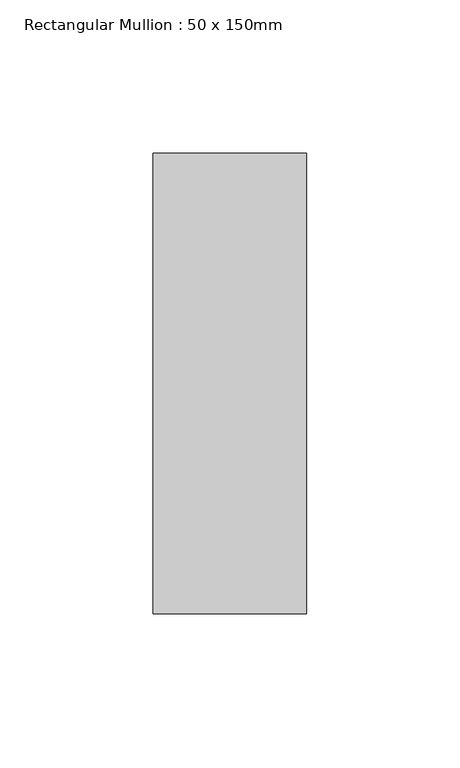
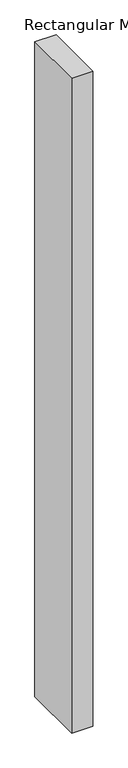
"""IFC4 building model written with IfcOpenShell, lengths in millimetres: member geometry, Rectangular Mullion : 50 x 150mm."""

from ifc_helpers import new_model, si_unit, frame, origin, place, context, project, spatial, polyline, outline, extrude, source, transform, mapped, element, save


def rectangular_mullion_50_x_150mm_9bc3b149(model_context):
    return source(origin(), model_context, "Body", "SweptSolid", [
        extrude(outline(polyline([(25.0, 75.0), (25.0, -75.0), (-25.0, -75.0), (-25.0, 75.0), (25.0, 75.0)])), frame((0.0, 0.0, -1635.0991456), z_axis=(0.0, 0.0, 1.0), x_axis=(1.0, 0.0, 0.0)), (0.0, 0.0, 1.0), 1635.0991456),
    ])


if __name__ == "__main__":
    model = new_model("IFC4")
    model_context = context("Model", 3, world=origin())
    ifc_project = project(units=[si_unit("LENGTHUNIT", "METRE", prefix="MILLI")], contexts=[model_context])
    site = spatial("IfcSite", under=ifc_project)
    building = spatial("IfcBuilding", under=site)
    placement = place(None, origin())
    rectangular_mullion_50_x_150mm_shape = rectangular_mullion_50_x_150mm_9bc3b149(model_context)
    element("IfcMember", 1, ObjectType="Rectangular Mullion : 50 x 150mm", at=placement, inside=building, context=model_context, shape_type="MappedRepresentation", body=[
        mapped(rectangular_mullion_50_x_150mm_shape, transform((0.0, 0.0, 0.0), x_axis=(1.0, 0.0, 0.0), y_axis=(0.0, 1.0, 0.0), z_axis=(0.0, 0.0, 1.0))),
    ])
    save(model, "model.ifc")

# Revit data of these elements
# Type "Rectangular Mullion : 50 x 150mm"
#   built-in parameter 1007304 = 0.492126 (stored number, unit not read)
#   built-in parameter 1007301 = 0.082021 (stored number, unit not read)
#   built-in parameter 1007300 = 0.082021 (stored number, unit not read)
# Element 1 (IfcMember, "Rectangular Mullion : 50 x 150mm")
#   Materials on its faces: "Aluminium"
# Materials
#   "Aluminium": class "Metal", colour RGB 247 247 247, transparency 0, Description = "Aluminium 6061", Cost = 0
